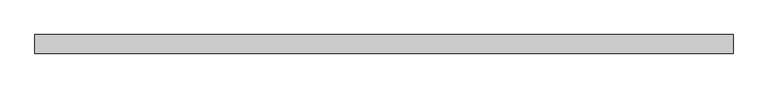
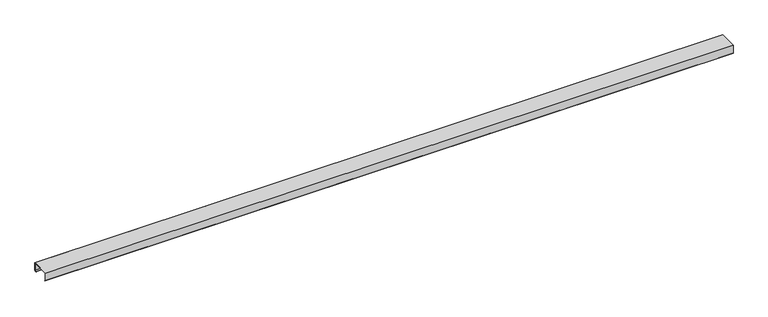
"""IFC4 building model written with IfcOpenShell, lengths in millimetres: proxy geometry, Generic Models 7:Generic Models 1:1:Generic Models 1:1 : Generic Models 7:Generic Models 1:337419:1 : Generic Models 7:Generic Models 1:1:Generic Models 1:1 : Generic Models 7:Generic Models 1:337419:306201."""

from ifc_helpers import new_model, si_unit, frame, origin, place, context, project, spatial, polyline, outline, extrude, source, transform, mapped, element, save


def generic_models_480be813(model_context):
    return source(origin(), model_context, "Body", "SweptSolid", [
        extrude(outline(polyline([(-579000.6913841, 1309.4890625), (-578797.4913841, 1309.4890625), (-578797.4913841, 1220.5890625), (-578812.0845307, 1208.3439586), (-578813.8702751, 1210.4721258), (-578800.2695091, 1221.8845235), (-578800.2695091, 1306.7109375), (-578997.9132591, 1306.7109375), (-578997.9132591, 1221.8845235), (-578984.3124931, 1210.4721258), (-578986.0982375, 1208.3439586), (-579000.6913841, 1220.5890625), (-579000.6913841, 1309.4890625)])), frame((588867.6367239, 0.0, 0.0), z_axis=(1.0, 0.0, 0.0), x_axis=(0.0, 1.0, 0.0)), (0.0, 0.0, 1.0), 7624.2408597),
    ])


if __name__ == "__main__":
    model = new_model("IFC4")
    model_context = context("Model", 3, world=origin())
    ifc_project = project(units=[si_unit("LENGTHUNIT", "METRE", prefix="MILLI")], contexts=[model_context])
    site = spatial("IfcSite", under=ifc_project)
    building = spatial("IfcBuilding", under=site)
    placement = place(None, origin())
    generic_models_shape = generic_models_480be813(model_context)
    element("IfcBuildingElementProxy", 1, Name="Generic Models 7:Generic Models 1:1:Generic Models 1:1 : Generic Models 7:Generic Models 1:337419:1 : Generic Models 7:Generic Models 1:1:Generic Models 1:1 : Generic Models 7:Generic Models 1:337419:306201", ObjectType="Generic Models 7:Generic Models 1:1:Generic Models 1:1 : Generic Models 7:Generic Models 1:337419:1 : Generic Models 7:Generic Models 1:1:Generic Models 1:1 : Generic Models 7:Generic Models 1:337419:306201", at=placement, inside=building, context=model_context, shape_type="MappedRepresentation", body=[
        mapped(generic_models_shape, transform((0.0, 0.0, 0.0), x_axis=(1.0, 0.0, 0.0), y_axis=(0.0, 1.0, 0.0), z_axis=(0.0, 0.0, 1.0))),
    ])
    save(model, "model.ifc")

# Revit data of these elements
# Type "Generic Models 7:Generic Models 1:1:Generic Models 1:1 : Generic Models 7:Generic Models 1:337419:1 : Generic Models 7:Generic Models 1:1:Generic Models 1:1 : Generic Models 7:Generic Models 1:337419:306201"
#   NameOverride = "Generic Models 7:Generic Models 1:1:Generic Models 1:1 : Generic Models 7:Generic Models 1:337419:306201"
#   ObjectTypeOverride = "Generic Models 1:1 : Generic Models 7:Generic Models 1:337419"
#   Reference = "Generic Models 1"
#   Tag = "306201"
# Element 1 (IfcBuildingElementProxy, "Generic Models 7:Generic Models 1:1:Generic Models 1:1 : Generic Models 7:Generic Models 1:337419:1 : Generic Models 7:Generic Models 1:1:Generic Models 1:1 : Generic Models 7:Generic Models 1:337419:306201")
#   Materials on its faces: "CEE' SECTION (8.0x3.5C - SEE STRUCT. DWGS)"
# Materials
#   "CEE' SECTION (8.0x3.5C - SEE STRUCT. DWGS)": class "Unassigned", colour RGB 210 209 208, transparency 0, Keynote = "M05121300.02", Cost = 0
